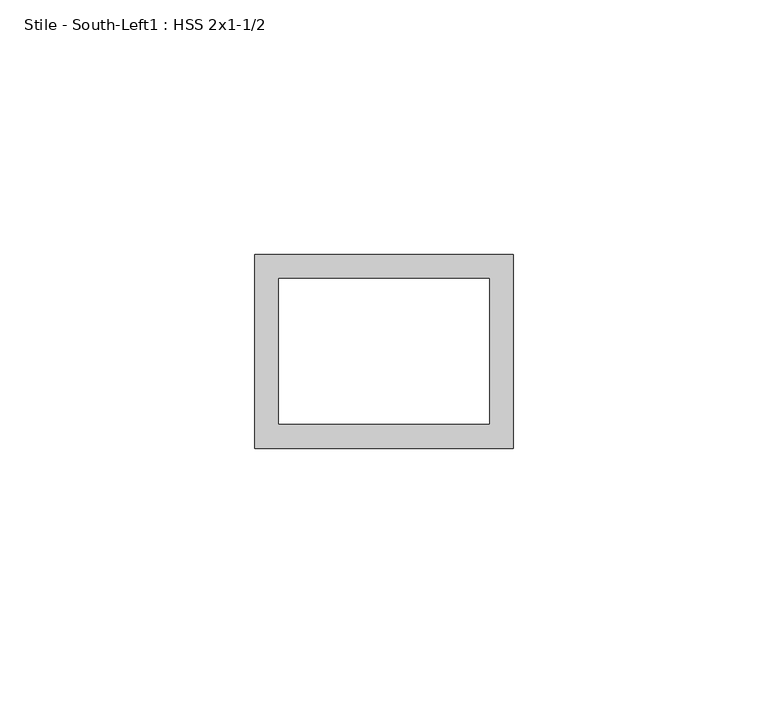
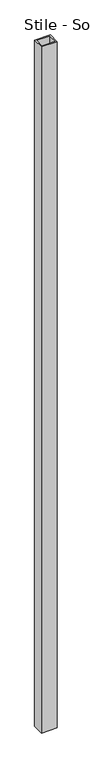
"""IFC4 building model written with IfcOpenShell, lengths in millimetres: proxy geometry, Stile - South-Left1 : HSS 2x1-1/2."""

from ifc_helpers import new_model, si_unit, frame, origin, place, context, project, spatial, polyline, outline, extrude, source, transform, mapped, element, save


def stile_south_left1_hss_2x1_1_2_18bcf153(model_context):
    return source(origin(), model_context, "Body", "SweptSolid", [
        extrude(outline(polyline([(587365.8934739, -535207.9163841), (587416.6934739, -535207.9163841), (587416.6934739, -535246.0163841), (587365.8934739, -535246.0163841), (587365.8934739, -535207.9163841)]), holes=[polyline([(587370.6559739, -535212.6788841), (587370.6559739, -535241.2538841), (587411.9309739, -535241.2538841), (587411.9309739, -535212.6788841), (587370.6559739, -535212.6788841)])]), frame((0.0, 0.0, 50.8), z_axis=(0.0, 0.0, 1.0), x_axis=(1.0, 0.0, 0.0)), (0.0, 0.0, 1.0), 2349.5),
    ])


if __name__ == "__main__":
    model = new_model("IFC4")
    model_context = context("Model", 3, world=origin())
    ifc_project = project(units=[si_unit("LENGTHUNIT", "METRE", prefix="MILLI")], contexts=[model_context])
    site = spatial("IfcSite", under=ifc_project)
    building = spatial("IfcBuilding", under=site)
    placement = place(None, origin())
    stile_south_left1_hss_2x1_1_2_shape = stile_south_left1_hss_2x1_1_2_18bcf153(model_context)
    element("IfcBuildingElementProxy", 1, Name="Stile - South-Left1 : HSS 2x1-1/2", ObjectType="Stile - South-Left1 : HSS 2x1-1/2", at=placement, inside=building, context=model_context, shape_type="MappedRepresentation", body=[
        mapped(stile_south_left1_hss_2x1_1_2_shape, transform((0.0, 0.0, 0.0), x_axis=(1.0, 0.0, 0.0), y_axis=(0.0, 1.0, 0.0), z_axis=(0.0, 0.0, 1.0))),
    ])
    save(model, "model.ifc")

# Revit data of these elements
# Element 1 (IfcBuildingElementProxy, "Stile - South-Left1 : HSS 2x1-1/2")
#   Materials on its faces: "1-1/2\"X2\" GALV. STL HSS TUBING"
# Materials
#   "1-1/2\"X2\" GALV. STL HSS TUBING": class "Generic", colour RGB 211 211 207, transparency 0, Cost = 0
